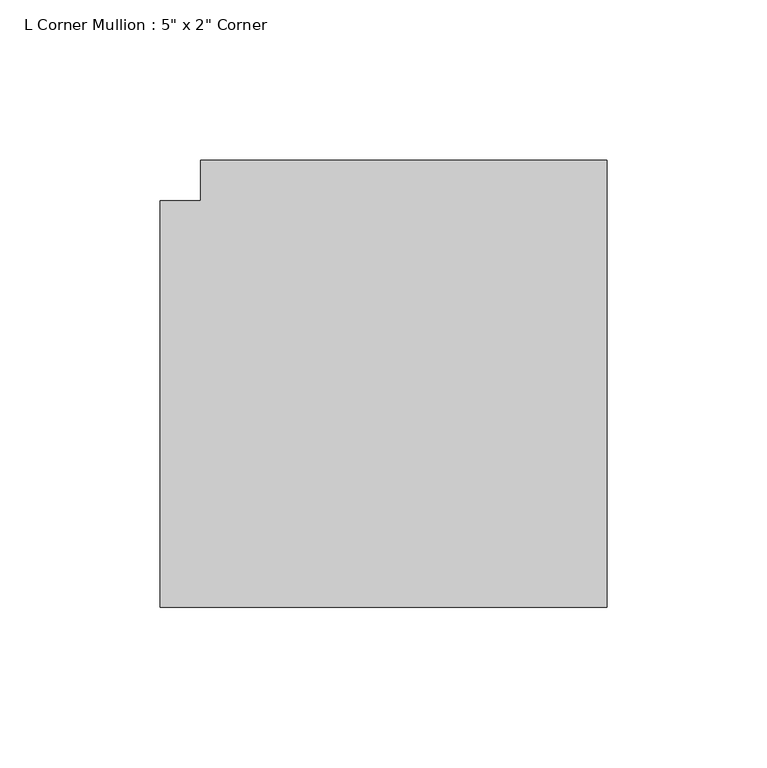
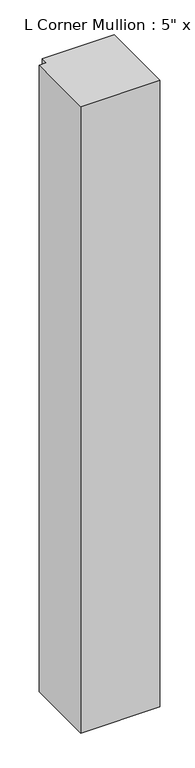
"""IFC4 building model written with IfcOpenShell, lengths in millimetres: member geometry."""

from ifc_helpers import new_model, si_unit, frame, origin, place, context, project, spatial, polyline, outline, extrude, source, transform, mapped, element, save


def member_390eb7cd(model_context):
    return source(origin(), model_context, "Body", "SweptSolid", [
        extrude(outline(polyline([(63.5, 76.2), (63.5, -63.5), (-76.2, -63.5), (-76.2, 63.5), (-63.5, 63.5), (-63.5, 76.2), (63.5, 76.2)])), frame((0.0, 0.0, -1168.4), z_axis=(0.0, 0.0, 1.0), x_axis=(1.0, 0.0, 0.0)), (0.0, 0.0, 1.0), 1168.4),
    ])


if __name__ == "__main__":
    model = new_model("IFC4")
    model_context = context("Model", 3, world=origin())
    ifc_project = project(units=[si_unit("LENGTHUNIT", "METRE", prefix="MILLI")], contexts=[model_context])
    site = spatial("IfcSite", under=ifc_project)
    building = spatial("IfcBuilding", under=site)
    placement = place(None, origin())
    member_shape = member_390eb7cd(model_context)
    element("IfcMember", 1, ObjectType="L Corner Mullion : 5\" x 2\" Corner", at=placement, inside=building, context=model_context, shape_type="MappedRepresentation", body=[
        mapped(member_shape, transform((0.0, 0.0, 0.0), x_axis=(1.0, 0.0, 0.0), y_axis=(0.0, 1.0, 0.0), z_axis=(0.0, 0.0, 1.0))),
    ])
    save(model, "model.ifc")

# Revit data of these elements
# Project information
#   Project Issue Date = "Issue Date"
#   Project Status = "Project Status"
#   Client Name = "Owner"
#   Project Address = "Enter address here"
#   Project Name = "Project Name"
#   Project Number = "Project Number"
# Type "L Corner Mullion : 5\" x 2\" Corner"
#   built-in parameter 1007355 = 0.25 (stored number, unit not read)
#   built-in parameter 1007354 = 0.25 (stored number, unit not read)
#   built-in parameter 1007304 = 0.416667 (stored number, unit not read)
# Element 1 (IfcMember, "L Corner Mullion : 5\" x 2\" Corner")
#   Materials on its faces: "Metal - Aluminum"
# Materials
#   "Metal - Aluminum": class "Metal", colour RGB 109 108 108, transparency 0
